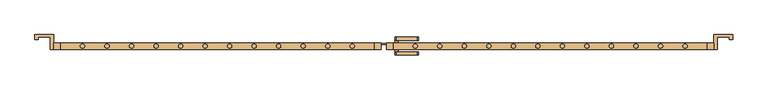
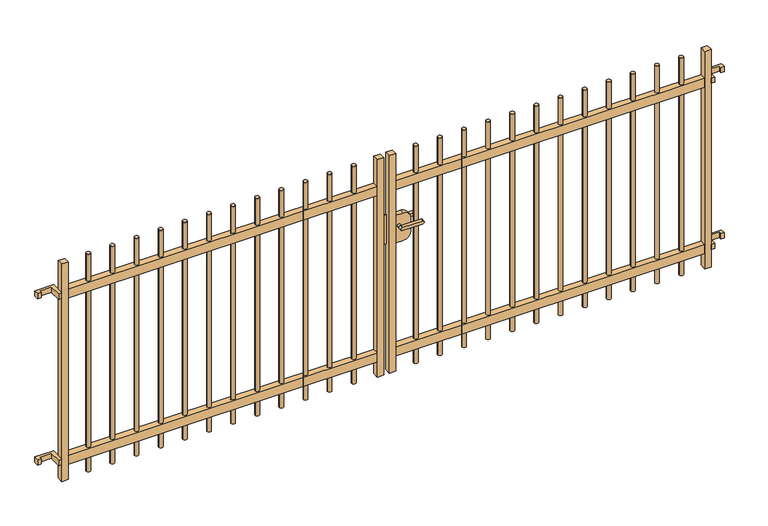
"""IFC4 building model written with IfcOpenShell, lengths in millimetres: door geometry, NLRS_90_DO_UN_draaipoort met spijlen 4000x1500_gen_rsf : draaipoort bxh 4000x1500mm-NP."""

from ifc_helpers import new_model, si_unit, point, frame, frame_2d, origin, place, context, project, spatial, polyline, circle_curve, trimmed, segment, composite_curve, outline, extrude, source, transform, mapped, element, save


def door_459dbaae(model_context):
    return source(origin(), model_context, "Body", "SweptSolid", [
        extrude(outline(composite_curve([segment(trimmed(circle_curve(frame_2d((-1842.5, 0.0)), 13.0), [point((-1855.5, 1.1e-06))], [point((-1829.5, -1.1e-06))], False, "CARTESIAN"), True, "CONTINUOUS"), segment(trimmed(circle_curve(frame_2d((-1842.5, 0.0)), 13.0), [point((-1829.5, -1.1e-06))], [point((-1855.5, 1.1e-06))], False, "CARTESIAN"), True, "CONTINUOUS")], self_intersect=False)), frame((0.0, 0.0, 50.0), z_axis=(0.0, 0.0, 1.0), x_axis=(1.0, 0.0, 0.0)), (0.0, 0.0, 1.0), 1430.0),
        extrude(outline(composite_curve([segment(trimmed(circle_curve(frame_2d((-1692.5, 0.0)), 13.0), [point((-1705.5, 1.1e-06))], [point((-1679.5, -1.1e-06))], False, "CARTESIAN"), True, "CONTINUOUS"), segment(trimmed(circle_curve(frame_2d((-1692.5, 0.0)), 13.0), [point((-1679.5, -1.1e-06))], [point((-1705.5, 1.1e-06))], False, "CARTESIAN"), True, "CONTINUOUS")], self_intersect=False)), frame((0.0, 0.0, 50.0), z_axis=(0.0, 0.0, 1.0), x_axis=(1.0, 0.0, 0.0)), (0.0, 0.0, 1.0), 1430.0),
        extrude(outline(composite_curve([segment(trimmed(circle_curve(frame_2d((-1542.5, 0.0)), 13.0), [point((-1555.5, 1.1e-06))], [point((-1529.5, -1.1e-06))], False, "CARTESIAN"), True, "CONTINUOUS"), segment(trimmed(circle_curve(frame_2d((-1542.5, 0.0)), 13.0), [point((-1529.5, -1.1e-06))], [point((-1555.5, 1.1e-06))], False, "CARTESIAN"), True, "CONTINUOUS")], self_intersect=False)), frame((0.0, 0.0, 50.0), z_axis=(0.0, 0.0, 1.0), x_axis=(1.0, 0.0, 0.0)), (0.0, 0.0, 1.0), 1430.0),
        extrude(outline(composite_curve([segment(trimmed(circle_curve(frame_2d((-1392.5, 0.0)), 13.0), [point((-1405.5, 1.1e-06))], [point((-1379.5, -1.1e-06))], False, "CARTESIAN"), True, "CONTINUOUS"), segment(trimmed(circle_curve(frame_2d((-1392.5, 0.0)), 13.0), [point((-1379.5, -1.1e-06))], [point((-1405.5, 1.1e-06))], False, "CARTESIAN"), True, "CONTINUOUS")], self_intersect=False)), frame((0.0, 0.0, 50.0), z_axis=(0.0, 0.0, 1.0), x_axis=(1.0, 0.0, 0.0)), (0.0, 0.0, 1.0), 1430.0),
        extrude(outline(composite_curve([segment(trimmed(circle_curve(frame_2d((-1242.5, 0.0)), 13.0), [point((-1255.5, 1.1e-06))], [point((-1229.5, -1.1e-06))], False, "CARTESIAN"), True, "CONTINUOUS"), segment(trimmed(circle_curve(frame_2d((-1242.5, 0.0)), 13.0), [point((-1229.5, -1.1e-06))], [point((-1255.5, 1.1e-06))], False, "CARTESIAN"), True, "CONTINUOUS")], self_intersect=False)), frame((0.0, 0.0, 50.0), z_axis=(0.0, 0.0, 1.0), x_axis=(1.0, 0.0, 0.0)), (0.0, 0.0, 1.0), 1430.0),
        extrude(outline(composite_curve([segment(trimmed(circle_curve(frame_2d((-1092.5, 0.0)), 13.0), [point((-1105.5, 1.1e-06))], [point((-1079.5, -1.1e-06))], False, "CARTESIAN"), True, "CONTINUOUS"), segment(trimmed(circle_curve(frame_2d((-1092.5, 0.0)), 13.0), [point((-1079.5, -1.1e-06))], [point((-1105.5, 1.1e-06))], False, "CARTESIAN"), True, "CONTINUOUS")], self_intersect=False)), frame((0.0, 0.0, 50.0), z_axis=(0.0, 0.0, 1.0), x_axis=(1.0, 0.0, 0.0)), (0.0, 0.0, 1.0), 1430.0),
        extrude(outline(composite_curve([segment(trimmed(circle_curve(frame_2d((-942.5, 0.0)), 13.0), [point((-955.5, 1.1e-06))], [point((-929.5, -1.1e-06))], False, "CARTESIAN"), True, "CONTINUOUS"), segment(trimmed(circle_curve(frame_2d((-942.5, 0.0)), 13.0), [point((-929.5, -1.1e-06))], [point((-955.5, 1.1e-06))], False, "CARTESIAN"), True, "CONTINUOUS")], self_intersect=False)), frame((0.0, 0.0, 50.0), z_axis=(0.0, 0.0, 1.0), x_axis=(1.0, 0.0, 0.0)), (0.0, 0.0, 1.0), 1430.0),
        extrude(outline(composite_curve([segment(trimmed(circle_curve(frame_2d((-792.5, 0.0)), 13.0), [point((-805.5, 1.1e-06))], [point((-779.5, -1.1e-06))], False, "CARTESIAN"), True, "CONTINUOUS"), segment(trimmed(circle_curve(frame_2d((-792.5, 0.0)), 13.0), [point((-779.5, -1.1e-06))], [point((-805.5, 1.1e-06))], False, "CARTESIAN"), True, "CONTINUOUS")], self_intersect=False)), frame((0.0, 0.0, 50.0), z_axis=(0.0, 0.0, 1.0), x_axis=(1.0, 0.0, 0.0)), (0.0, 0.0, 1.0), 1430.0),
        extrude(outline(composite_curve([segment(trimmed(circle_curve(frame_2d((-642.5, 0.0)), 13.0), [point((-655.5, 1.1e-06))], [point((-629.5, -1.1e-06))], False, "CARTESIAN"), True, "CONTINUOUS"), segment(trimmed(circle_curve(frame_2d((-642.5, 0.0)), 13.0), [point((-629.5, -1.1e-06))], [point((-655.5, 1.1e-06))], False, "CARTESIAN"), True, "CONTINUOUS")], self_intersect=False)), frame((0.0, 0.0, 50.0), z_axis=(0.0, 0.0, 1.0), x_axis=(1.0, 0.0, 0.0)), (0.0, 0.0, 1.0), 1430.0),
        extrude(outline(composite_curve([segment(trimmed(circle_curve(frame_2d((-192.5, 0.0)), 13.0), [point((-205.5, 1.1e-06))], [point((-179.5, -1.1e-06))], False, "CARTESIAN"), True, "CONTINUOUS"), segment(trimmed(circle_curve(frame_2d((-192.5, 0.0)), 13.0), [point((-179.5, -1.1e-06))], [point((-205.5, 1.1e-06))], False, "CARTESIAN"), True, "CONTINUOUS")], self_intersect=False)), frame((0.0, 0.0, 50.0), z_axis=(0.0, 0.0, 1.0), x_axis=(1.0, 0.0, 0.0)), (0.0, 0.0, 1.0), 1430.0),
        extrude(outline(composite_curve([segment(trimmed(circle_curve(frame_2d((-342.5, 0.0)), 13.0), [point((-355.5, 1.1e-06))], [point((-329.5, -1.1e-06))], False, "CARTESIAN"), True, "CONTINUOUS"), segment(trimmed(circle_curve(frame_2d((-342.5, 0.0)), 13.0), [point((-329.5, -1.1e-06))], [point((-355.5, 1.1e-06))], False, "CARTESIAN"), True, "CONTINUOUS")], self_intersect=False)), frame((0.0, 0.0, 50.0), z_axis=(0.0, 0.0, 1.0), x_axis=(1.0, 0.0, 0.0)), (0.0, 0.0, 1.0), 1430.0),
        extrude(outline(composite_curve([segment(trimmed(circle_curve(frame_2d((-492.5, 0.0)), 13.0), [point((-505.5, 1.1e-06))], [point((-479.5, -1.1e-06))], False, "CARTESIAN"), True, "CONTINUOUS"), segment(trimmed(circle_curve(frame_2d((-492.5, 0.0)), 13.0), [point((-479.5, -1.1e-06))], [point((-505.5, 1.1e-06))], False, "CARTESIAN"), True, "CONTINUOUS")], self_intersect=False)), frame((0.0, 0.0, 50.0), z_axis=(0.0, 0.0, 1.0), x_axis=(1.0, 0.0, 0.0)), (0.0, 0.0, 1.0), 1430.0),
        extrude(outline(polyline([(-1977.5, -20.0), (-2017.5, -20.0), (-2017.5, 20.0), (-1977.5, 20.0), (-1977.5, -20.0)])), frame((0.0, 0.0, 50.0), z_axis=(0.0, 0.0, 1.0), x_axis=(1.0, 0.0, 0.0)), (0.0, 0.0, 1.0), 1430.0),
        extrude(outline(polyline([(-17.5, -20.0), (-57.5, -20.0), (-57.5, 20.0), (-17.5, 20.0), (-17.5, -20.0)])), frame((0.0, 0.0, 50.0), z_axis=(0.0, 0.0, 1.0), x_axis=(1.0, 0.0, 0.0)), (0.0, 0.0, 1.0), 1430.0),
        extrude(outline(composite_curve([segment(trimmed(circle_curve(frame_2d((1842.5, 0.0)), 13.0), [point((1855.5, 0.0))], [point((1829.5, 0.0))], False, "CARTESIAN"), True, "CONTINUOUS"), segment(trimmed(circle_curve(frame_2d((1842.5, 0.0)), 13.0), [point((1829.5, 0.0))], [point((1855.5, 0.0))], False, "CARTESIAN"), True, "CONTINUOUS")], self_intersect=False)), frame((0.0, 0.0, 50.0), z_axis=(0.0, 0.0, 1.0), x_axis=(1.0, 0.0, 0.0)), (0.0, 0.0, 1.0), 1430.0),
        extrude(outline(composite_curve([segment(trimmed(circle_curve(frame_2d((1692.5, 0.0)), 13.0), [point((1705.5, 0.0))], [point((1679.5, 0.0))], False, "CARTESIAN"), True, "CONTINUOUS"), segment(trimmed(circle_curve(frame_2d((1692.5, 0.0)), 13.0), [point((1679.5, 0.0))], [point((1705.5, 0.0))], False, "CARTESIAN"), True, "CONTINUOUS")], self_intersect=False)), frame((0.0, 0.0, 50.0), z_axis=(0.0, 0.0, 1.0), x_axis=(1.0, 0.0, 0.0)), (0.0, 0.0, 1.0), 1430.0),
        extrude(outline(composite_curve([segment(trimmed(circle_curve(frame_2d((1542.5, 0.0)), 13.0), [point((1555.5, 0.0))], [point((1529.5, 0.0))], False, "CARTESIAN"), True, "CONTINUOUS"), segment(trimmed(circle_curve(frame_2d((1542.5, 0.0)), 13.0), [point((1529.5, 0.0))], [point((1555.5, 0.0))], False, "CARTESIAN"), True, "CONTINUOUS")], self_intersect=False)), frame((0.0, 0.0, 50.0), z_axis=(0.0, 0.0, 1.0), x_axis=(1.0, 0.0, 0.0)), (0.0, 0.0, 1.0), 1430.0),
        extrude(outline(composite_curve([segment(trimmed(circle_curve(frame_2d((1392.5, 0.0)), 13.0), [point((1405.5, 0.0))], [point((1379.5, 0.0))], False, "CARTESIAN"), True, "CONTINUOUS"), segment(trimmed(circle_curve(frame_2d((1392.5, 0.0)), 13.0), [point((1379.5, 0.0))], [point((1405.5, 0.0))], False, "CARTESIAN"), True, "CONTINUOUS")], self_intersect=False)), frame((0.0, 0.0, 50.0), z_axis=(0.0, 0.0, 1.0), x_axis=(1.0, 0.0, 0.0)), (0.0, 0.0, 1.0), 1430.0),
        extrude(outline(composite_curve([segment(trimmed(circle_curve(frame_2d((1242.5, 0.0)), 13.0), [point((1255.5, 0.0))], [point((1229.5, 0.0))], False, "CARTESIAN"), True, "CONTINUOUS"), segment(trimmed(circle_curve(frame_2d((1242.5, 0.0)), 13.0), [point((1229.5, 0.0))], [point((1255.5, 0.0))], False, "CARTESIAN"), True, "CONTINUOUS")], self_intersect=False)), frame((0.0, 0.0, 50.0), z_axis=(0.0, 0.0, 1.0), x_axis=(1.0, 0.0, 0.0)), (0.0, 0.0, 1.0), 1430.0),
        extrude(outline(composite_curve([segment(trimmed(circle_curve(frame_2d((1092.5, 0.0)), 13.0), [point((1105.5, 0.0))], [point((1079.5, 0.0))], False, "CARTESIAN"), True, "CONTINUOUS"), segment(trimmed(circle_curve(frame_2d((1092.5, 0.0)), 13.0), [point((1079.5, 0.0))], [point((1105.5, 0.0))], False, "CARTESIAN"), True, "CONTINUOUS")], self_intersect=False)), frame((0.0, 0.0, 50.0), z_axis=(0.0, 0.0, 1.0), x_axis=(1.0, 0.0, 0.0)), (0.0, 0.0, 1.0), 1430.0),
        extrude(outline(composite_curve([segment(trimmed(circle_curve(frame_2d((942.5, 0.0)), 13.0), [point((955.5, 0.0))], [point((929.5, 0.0))], False, "CARTESIAN"), True, "CONTINUOUS"), segment(trimmed(circle_curve(frame_2d((942.5, 0.0)), 13.0), [point((929.5, 0.0))], [point((955.5, 0.0))], False, "CARTESIAN"), True, "CONTINUOUS")], self_intersect=False)), frame((0.0, 0.0, 50.0), z_axis=(0.0, 0.0, 1.0), x_axis=(1.0, 0.0, 0.0)), (0.0, 0.0, 1.0), 1430.0),
        extrude(outline(composite_curve([segment(trimmed(circle_curve(frame_2d((792.5, 0.0)), 13.0), [point((805.5, 0.0))], [point((779.5, 0.0))], False, "CARTESIAN"), True, "CONTINUOUS"), segment(trimmed(circle_curve(frame_2d((792.5, 0.0)), 13.0), [point((779.5, 0.0))], [point((805.5, 0.0))], False, "CARTESIAN"), True, "CONTINUOUS")], self_intersect=False)), frame((0.0, 0.0, 50.0), z_axis=(0.0, 0.0, 1.0), x_axis=(1.0, 0.0, 0.0)), (0.0, 0.0, 1.0), 1430.0),
        extrude(outline(composite_curve([segment(trimmed(circle_curve(frame_2d((642.5, 0.0)), 13.0), [point((655.5, 0.0))], [point((629.5, 0.0))], False, "CARTESIAN"), True, "CONTINUOUS"), segment(trimmed(circle_curve(frame_2d((642.5, 0.0)), 13.0), [point((629.5, 0.0))], [point((655.5, 0.0))], False, "CARTESIAN"), True, "CONTINUOUS")], self_intersect=False)), frame((0.0, 0.0, 50.0), z_axis=(0.0, 0.0, 1.0), x_axis=(1.0, 0.0, 0.0)), (0.0, 0.0, 1.0), 1430.0),
        extrude(outline(composite_curve([segment(trimmed(circle_curve(frame_2d((192.5, 0.0)), 13.0), [point((205.5, 0.0))], [point((179.5, 0.0))], False, "CARTESIAN"), True, "CONTINUOUS"), segment(trimmed(circle_curve(frame_2d((192.5, 0.0)), 13.0), [point((179.5, 0.0))], [point((205.5, 0.0))], False, "CARTESIAN"), True, "CONTINUOUS")], self_intersect=False)), frame((0.0, 0.0, 50.0), z_axis=(0.0, 0.0, 1.0), x_axis=(1.0, 0.0, 0.0)), (0.0, 0.0, 1.0), 1430.0),
        extrude(outline(composite_curve([segment(trimmed(circle_curve(frame_2d((342.5, 0.0)), 13.0), [point((355.5, 0.0))], [point((329.5, 0.0))], False, "CARTESIAN"), True, "CONTINUOUS"), segment(trimmed(circle_curve(frame_2d((342.5, 0.0)), 13.0), [point((329.5, 0.0))], [point((355.5, 0.0))], False, "CARTESIAN"), True, "CONTINUOUS")], self_intersect=False)), frame((0.0, 0.0, 50.0), z_axis=(0.0, 0.0, 1.0), x_axis=(1.0, 0.0, 0.0)), (0.0, 0.0, 1.0), 1430.0),
        extrude(outline(composite_curve([segment(trimmed(circle_curve(frame_2d((492.5, 0.0)), 13.0), [point((505.5, 0.0))], [point((479.5, 0.0))], False, "CARTESIAN"), True, "CONTINUOUS"), segment(trimmed(circle_curve(frame_2d((492.5, 0.0)), 13.0), [point((479.5, 0.0))], [point((505.5, 0.0))], False, "CARTESIAN"), True, "CONTINUOUS")], self_intersect=False)), frame((0.0, 0.0, 50.0), z_axis=(0.0, 0.0, 1.0), x_axis=(1.0, 0.0, 0.0)), (0.0, 0.0, 1.0), 1430.0),
        extrude(outline(polyline([(1977.5, -20.0), (1977.5, 20.0), (2017.5, 20.0), (2017.5, -20.0), (1977.5, -20.0)])), frame((0.0, 0.0, 50.0), z_axis=(0.0, 0.0, 1.0), x_axis=(1.0, 0.0, 0.0)), (0.0, 0.0, 1.0), 1430.0),
        extrude(outline(polyline([(17.5, -20.0), (17.5, 20.0), (57.5, 20.0), (57.5, -20.0), (17.5, -20.0)])), frame((0.0, 0.0, 50.0), z_axis=(0.0, 0.0, 1.0), x_axis=(1.0, 0.0, 0.0)), (0.0, 0.0, 1.0), 1430.0),
        extrude(outline(composite_curve([segment(polyline([(1008.625, 203.3906246), (1008.625, 78.3906258)]), True, "CONTINUOUS"), segment(trimmed(circle_curve(frame_2d((998.625, 78.390625)), 10.0), [point((1008.625, 78.3906258))], [point((988.625, 78.390625))], False, "CARTESIAN"), True, "CONTINUOUS"), segment(polyline([(988.625, 78.390625), (988.625, 203.3906269)]), True, "CONTINUOUS"), segment(trimmed(circle_curve(frame_2d((998.625, 203.390625)), 10.0), [point((988.625, 203.3906269))], [point((1008.625, 203.3906246))], False, "CARTESIAN"), True, "CONTINUOUS")], self_intersect=False)), frame((0.0, 35.0, 0.0), z_axis=(0.0, 1.0, 0.0), x_axis=(0.0, 0.0, 1.0)), (0.0, 0.0, 1.0), 20.0),
        extrude(outline(composite_curve([segment(polyline([(1008.625, 203.3906246), (1008.625, 78.3906258)]), True, "CONTINUOUS"), segment(trimmed(circle_curve(frame_2d((998.625, 78.390625)), 10.0), [point((1008.625, 78.3906258))], [point((988.625, 78.390625))], False, "CARTESIAN"), True, "CONTINUOUS"), segment(polyline([(988.625, 78.390625), (988.625, 203.3906269)]), True, "CONTINUOUS"), segment(trimmed(circle_curve(frame_2d((998.625, 203.390625)), 10.0), [point((988.625, 203.3906269))], [point((1008.625, 203.3906246))], False, "CARTESIAN"), True, "CONTINUOUS")], self_intersect=False)), frame((0.0, -55.0, 0.0), z_axis=(0.0, 1.0, 0.0), x_axis=(0.0, 0.0, 1.0)), (0.0, 0.0, 1.0), 20.0),
        extrude(outline(polyline([(37.5, 10.0), (-17.5, 10.0), (-17.5, 15.0), (37.5, 15.0), (37.5, 10.0)])), frame((0.0, 0.0, 885.0625), z_axis=(0.0, 0.0, 1.0), x_axis=(1.0, 0.0, 0.0)), (0.0, 0.0, 1.0), 190.0),
        extrude(outline(composite_curve([segment(polyline([(1070.0, 57.5), (890.0, 57.5), (890.0, 107.499998)]), True, "CONTINUOUS"), segment(trimmed(circle_curve(frame_2d((935.0, 107.5)), 45.0), [point((890.0, 107.499998))], [point((935.0, 152.5))], False, "CARTESIAN"), True, "CONTINUOUS"), segment(polyline([(935.0, 152.5), (1025.0, 152.5)]), True, "CONTINUOUS"), segment(trimmed(circle_curve(frame_2d((1025.0, 107.5)), 45.0), [point((1025.0, 152.5))], [point((1070.0, 107.5))], False, "CARTESIAN"), True, "CONTINUOUS"), segment(polyline([(1070.0, 107.5), (1070.0, 57.5)]), True, "CONTINUOUS")], self_intersect=False)), frame((0.0, -15.0, 0.0), z_axis=(0.0, 1.0, 0.0), x_axis=(0.0, 0.0, 1.0)), (0.0, 0.0, 1.0), 30.0),
        extrude(outline(composite_curve([segment(trimmed(circle_curve(frame_2d((998.625, 78.390625)), 10.0), [point((998.6250009, 68.390625))], [point((998.6249991, 88.390625))], False, "CARTESIAN"), True, "CONTINUOUS"), segment(trimmed(circle_curve(frame_2d((998.625, 78.390625)), 10.0), [point((998.6249991, 88.390625))], [point((998.6250009, 68.390625))], False, "CARTESIAN"), True, "CONTINUOUS")], self_intersect=False)), frame((0.0, 15.0, 0.0), z_axis=(0.0, 1.0, 0.0), x_axis=(0.0, 0.0, 1.0)), (0.0, 0.0, 1.0), 20.0),
        extrude(outline(composite_curve([segment(trimmed(circle_curve(frame_2d((998.625, 78.390625)), 10.0), [point((998.6250009, 68.390625))], [point((998.6249991, 88.390625))], False, "CARTESIAN"), True, "CONTINUOUS"), segment(trimmed(circle_curve(frame_2d((998.625, 78.390625)), 10.0), [point((998.6249991, 88.390625))], [point((998.6250009, 68.390625))], False, "CARTESIAN"), True, "CONTINUOUS")], self_intersect=False)), frame((0.0, -35.0, 0.0), z_axis=(0.0, 1.0, 0.0), x_axis=(0.0, 0.0, 1.0)), (0.0, 0.0, 1.0), 20.0),
        extrude(outline(polyline([(-2017.5, -20.0), (-2038.5, -20.0), (-2038.5, 56.65625), (-2112.25, 56.65625), (-2112.25, 40.0), (-2133.5, 40.0), (-2133.5, 70.0), (-2017.5, 70.0), (-2017.5, -20.0)])), frame((0.0, 0.0, 1256.1498273), z_axis=(0.0, 0.0, 1.0), x_axis=(1.0, 0.0, 0.0)), (0.0, 0.0, 1.0), 35.0),
        extrude(outline(polyline([(-57.5, -20.0), (-1977.5, -20.0), (-1977.5, 20.0), (-57.5, 20.0), (-57.5, -20.0)])), frame((0.0, 0.0, 1243.6498273), z_axis=(0.0, 0.0, 1.0), x_axis=(1.0, 0.0, 0.0)), (0.0, 0.0, 1.0), 60.0),
        extrude(outline(polyline([(-2017.5, -20.0), (-2038.5, -20.0), (-2038.5, 56.65625), (-2112.25, 56.65625), (-2112.25, 40.0), (-2133.5, 40.0), (-2133.5, 70.0), (-2017.5, 70.0), (-2017.5, -20.0)])), frame((0.0, 0.0, 162.5), z_axis=(0.0, 0.0, 1.0), x_axis=(1.0, 0.0, 0.0)), (0.0, 0.0, 1.0), 35.0),
        extrude(outline(polyline([(-57.5, -20.0), (-1977.5, -20.0), (-1977.5, 20.0), (-57.5, 20.0), (-57.5, -20.0)])), frame((0.0, 0.0, 150.0), z_axis=(0.0, 0.0, 1.0), x_axis=(1.0, 0.0, 0.0)), (0.0, 0.0, 1.0), 60.0),
        extrude(outline(polyline([(2017.5, -20.0), (2017.5, 70.0), (2133.5, 70.0), (2133.5, 40.0), (2112.25, 40.0), (2112.25, 56.65625), (2038.5, 56.65625), (2038.5, -20.0), (2017.5, -20.0)])), frame((0.0, 0.0, 1256.1498273), z_axis=(0.0, 0.0, 1.0), x_axis=(1.0, 0.0, 0.0)), (0.0, 0.0, 1.0), 35.0),
        extrude(outline(polyline([(57.5, -20.0), (57.5, 20.0), (1977.5, 20.0), (1977.5, -20.0), (57.5, -20.0)])), frame((0.0, 0.0, 1243.6498273), z_axis=(0.0, 0.0, 1.0), x_axis=(1.0, 0.0, 0.0)), (0.0, 0.0, 1.0), 60.0),
        extrude(outline(polyline([(2017.5, -20.0), (2017.5, 70.0), (2133.5, 70.0), (2133.5, 40.0), (2112.25, 40.0), (2112.25, 56.65625), (2038.5, 56.65625), (2038.5, -20.0), (2017.5, -20.0)])), frame((0.0, 0.0, 162.5), z_axis=(0.0, 0.0, 1.0), x_axis=(1.0, 0.0, 0.0)), (0.0, 0.0, 1.0), 35.0),
        extrude(outline(polyline([(57.5, -20.0), (57.5, 20.0), (1977.5, 20.0), (1977.5, -20.0), (57.5, -20.0)])), frame((0.0, 0.0, 150.0), z_axis=(0.0, 0.0, 1.0), x_axis=(1.0, 0.0, 0.0)), (0.0, 0.0, 1.0), 60.0),
    ])


if __name__ == "__main__":
    model = new_model("IFC4")
    model_context = context("Model", 3, world=origin())
    ifc_project = project(units=[si_unit("LENGTHUNIT", "METRE", prefix="MILLI")], contexts=[model_context])
    site = spatial("IfcSite", under=ifc_project)
    building = spatial("IfcBuilding", under=site)
    placement = place(None, origin())
    door_shape = door_459dbaae(model_context)
    element("IfcDoor", 1, ObjectType="NLRS_90_DO_UN_draaipoort met spijlen 4000x1500_gen_rsf : draaipoort bxh 4000x1500mm-NP", at=placement, inside=building, context=model_context, shape_type="MappedRepresentation", body=[
        mapped(door_shape, transform((0.0, 0.0, 0.0), x_axis=(1.0, 0.0, 0.0), y_axis=(0.0, 1.0, 0.0), z_axis=(0.0, 0.0, 1.0))),
    ])
    save(model, "model.ifc")

# Revit data of these elements
# Type "NLRS_90_DO_UN_draaipoort met spijlen 4000x1500_gen_rsf : draaipoort bxh 4000x1500mm-NP"
#   Type IfcGUID = "1A81voHkv98RYujw6ZYnw6"
#   IfcName[Type] = "draaipoort bxh 4000x1500mm-NP"
#   IfcDescription[Type] = "toegangspoort stalen spijlen bxh 4000x1500mm"
#   IfcExportAs[Type] = "IfcDoorType"
#   IfcExportType[Type] = "GATE"
#   NLRS_C_revit_versie = ""
#   NLRS_C_omschrijving_03 [instance default] = "doorgangsmaat"
#   NLRS_C_omschrijving_02 [instance default] = "sluiting"
#   NLRS_C_omschrijving_01 [instance default] = "poort"
#   NLRS_C_content_versie = ""
#   NLRS_C_content_provider = ""
#   NLRS_C_content_handleiding = ""
#   NLRS_C_content_datum_uitgifte = ""
#   NLRS_C_content_datum_gewijzigd = ""
#   NLRS_C_content_creator = ""
#   Model = "generiek"
#   Manufacturer = "Revit Standards Foundation"
#   Description = "toegangspoort stalen spijlen bxh 4000x1500mm"
#   Assembly Code = "90.32"
#   NLRS_C_hoogte = 1500.00 mm
#   NLRS_C_breedte_03 = 4130.00 mm
#   NLRS_C_breedte = 4165.00 mm
#   kolom rechts = no
#   kolom links = no
#   NLRS_C_materiaal_02 = NLRS_h_metaal_gen_rsf
#   NLRS_C_materiaal_01 = NLRS_h2_staal blauwgrijs_gen_rsf
#   URL = ""
#   Keynote = ""
#   Default Elevation = 0
# Element 1 (IfcDoor, "NLRS_90_DO_UN_draaipoort met spijlen 4000x1500_gen_rsf : draaipoort bxh 4000x1500mm-NP")
#   Materials on its faces: "NLRS_h2_staal blauwgrijs_gen_rsf", "NLRS_h_metaal_gen_rsf"
# Materials
#   "NLRS_h_metaal_gen_rsf": class "BCB class", colour RGB 149 148 153, transparency 0, Keynote = "h", Model = "generiek", Manufacturer = "Revit Standards Foundation", URL = "www.revitstandards.org", Description = "metaal", Cost = 0
#   "NLRS_h2_staal blauwgrijs_gen_rsf": class "BCB class", colour RGB 113 134 165, transparency 0, Keynote = "h2", Model = "generiek", Manufacturer = "Revit Standards Foundation", URL = "www.revitstandards.org", Description = "staal blauwgrijs", Cost = 0
